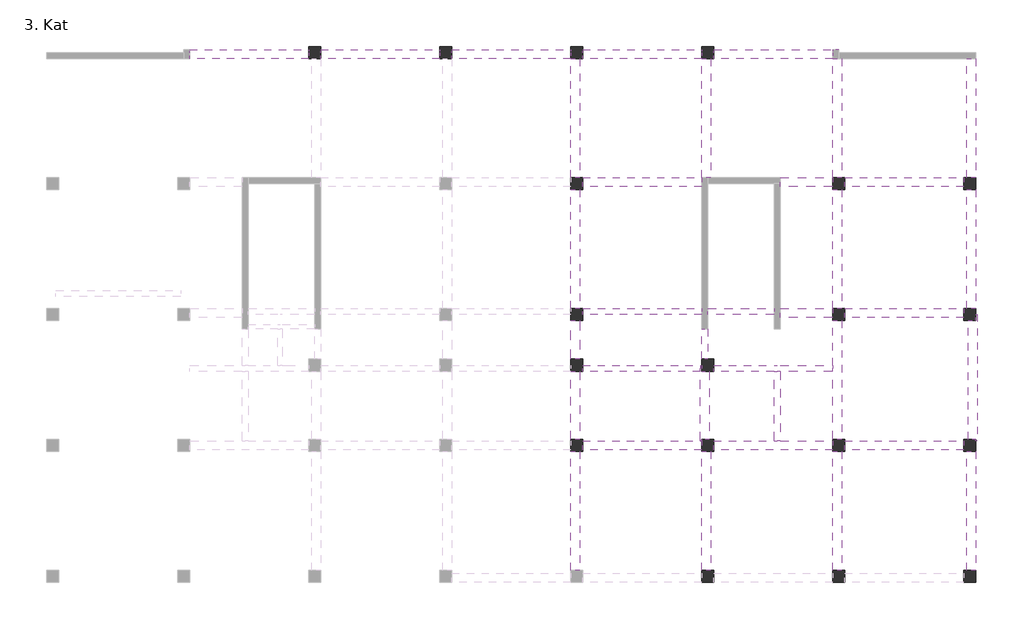
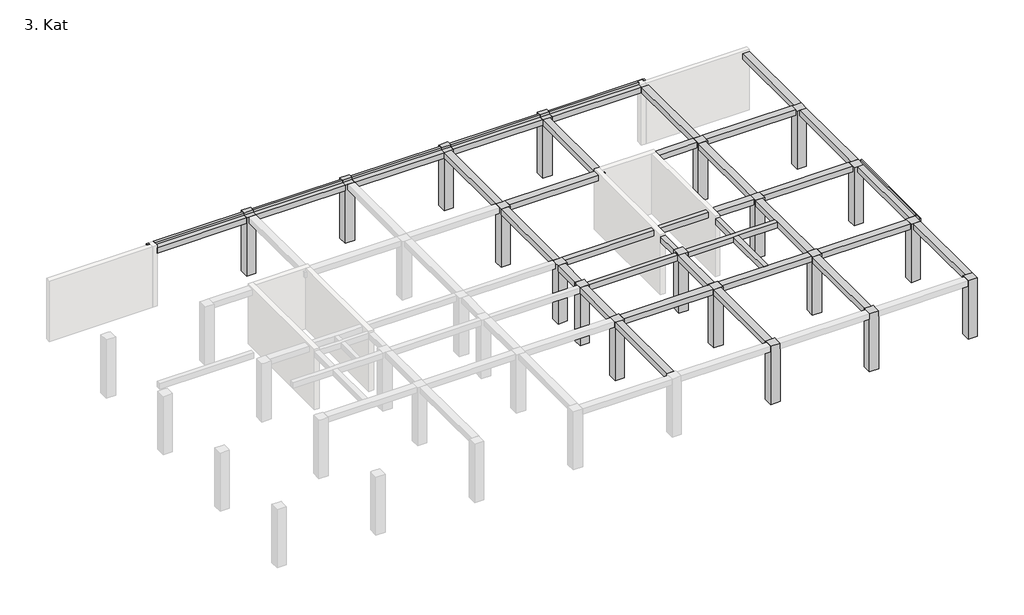
# One storey, part 2 of 2: 35 beams, 19 columns.
"""IFC4 building model written with IfcOpenShell, lengths in millimetres."""

from ifc_helpers import new_model, si_unit, frame, origin, place, context, project, spatial, polyline, outline, extrude, faceted_brep, element, save

model = new_model("IFC4")

# Units and contexts
model_context = context("Model", 3, world=origin())
ifc_project = project(units=[si_unit("LENGTHUNIT", "METRE", prefix="MILLI")], contexts=[model_context])

# Site, building, storey
site = spatial("IfcSite", under=ifc_project)
building = spatial("IfcBuilding", under=site)
storey = spatial("IfcBuildingStorey", under=building, Name="3. Kat", Elevation=15500.0)

# Beams
placement = place(None, origin())
element("IfcBeam", 1, ObjectType="M_Concrete-Rectangular Beam : 60x70cm kiriş", at=placement, inside=storey, context=model_context, shape_type="Brep", body=[
    faceted_brep([(16599.9993907, 34000.0004302, 21000.0), (16599.9993907, 34200.0000099, 21000.0), (8899.9995273, 34200.0000099, 21000.0), (8899.9995273, 34000.0004302, 21000.0), (8899.9993907, 33600.0000099, 20300.0), (16599.9993907, 33600.0000099, 20300.0), (16599.9993907, 33600.0000099, 20800.0), (8899.9993907, 33600.0000099, 20800.0), (8899.9995273, 34200.0000099, 20300.0), (16599.9993907, 34200.0000099, 20300.0), (8899.9993907, 34000.0004302, 20800.0), (16599.9993907, 34000.0004302, 20800.0)], [[[0, 1, 2, 3]], [[4, 5, 6, 7]], [[5, 4, 8, 9]], [[1, 9, 8, 2]], [[4, 7, 10, 3, 2, 8]], [[11, 10, 7, 6]], [[5, 9, 1, 0, 11, 6]], [[10, 11, 0, 3]]]),
    faceted_brep([(8299.9993907, 34200.0000099, 21000.0), (8299.9993907, 34200.0000099, 20300.0), (8299.9993907, 34000.0004302, 20300.0), (8299.9993907, 34000.0004302, 21000.0), (8499.9995273, 34000.0004302, 20300.0), (8499.9995273, 34000.0004302, 21000.0), (8499.9995273, 34200.0000099, 21000.0), (8499.9995273, 34200.0000099, 20300.0)], [[[0, 1, 2, 3]], [[3, 2, 4, 5]], [[6, 5, 4, 7]], [[0, 3, 5, 6]], [[2, 1, 7, 4]], [[1, 0, 6, 7]]]),
])
element("IfcBeam", 2, ObjectType="M_Concrete-Rectangular Beam : 60x70cm kiriş", at=placement, inside=storey, context=model_context, shape_type="SweptSolid", body=[
    extrude(outline(polyline([(34000.0004302, 21000.0), (34200.0000277, 21000.0), (34200.0000277, 20300.0), (33600.0000277, 20300.0), (33600.0000277, 20800.0), (34000.0004302, 20800.0), (34000.0004302, 21000.0)])), frame((17399.9993907, 0.0, 0.0), z_axis=(1.0, 0.0, 0.0), x_axis=(0.0, 1.0, 0.0)), (0.0, 0.0, 1.0), 7700.0),
])
element("IfcBeam", 3, ObjectType="M_Concrete-Rectangular Beam : 60x70cm kiriş", at=placement, inside=storey, context=model_context, shape_type="SweptSolid", body=[
    extrude(outline(polyline([(34000.0004302, 21000.0), (34200.000044, 21000.0), (34200.000044, 20300.0), (33600.000044, 20300.0), (33600.000044, 20800.0), (34000.0004302, 20800.0), (34000.0004302, 21000.0)])), frame((25899.9993907, 0.0, 0.0), z_axis=(1.0, 0.0, 0.0), x_axis=(0.0, 1.0, 0.0)), (0.0, 0.0, 1.0), 7700.0),
])
element("IfcBeam", 4, ObjectType="M_Concrete-Rectangular Beam : 60x70cm kiriş", at=placement, inside=storey, context=model_context, shape_type="SweptSolid", body=[
    extrude(outline(polyline([(34200.0000618, 21000.0), (34200.0000618, 20300.0), (33600.0000618, 20300.0), (33600.0000618, 20800.0), (34000.0004302, 20800.0), (34000.0004302, 21000.0), (34200.0000618, 21000.0)])), frame((34399.9993907, 0.0, 0.0), z_axis=(1.0, 0.0, 0.0), x_axis=(0.0, 1.0, 0.0)), (0.0, 0.0, 1.0), 7699.9999993),
])
element("IfcBeam", 5, ObjectType="M_Concrete-Rectangular Beam : 60x70cm kiriş", at=placement, inside=storey, context=model_context, shape_type="Brep", body=[
    faceted_brep([(50999.9994944, 34200.0000788, 21000.0), (42899.999681, 34200.0000788, 21000.0), (42899.999681, 34000.0004302, 21000.0), (50599.9994944, 34000.0004302, 21000.0), (50599.9994944, 34193.7257565, 21000.0), (50999.9994944, 34193.7257565, 21000.0), (50999.9994944, 34200.0000788, 20300.0), (42899.999681, 34200.0000788, 20300.0), (50999.9994944, 34193.7257565, 20300.0), (50599.9994944, 34193.7257565, 20300.0), (50599.9994944, 33600.0000788, 20300.0), (42899.999681, 33600.0000788, 20300.0), (42899.999681, 33600.0000788, 20800.0), (50599.9994944, 33600.0000788, 20800.0), (42899.999681, 34000.0004302, 20800.0), (50599.9994944, 34000.0004302, 20800.0)], [[[0, 1, 2, 3, 4, 5]], [[1, 0, 6, 7]], [[7, 6, 8, 9, 10, 11]], [[12, 11, 10, 13]], [[6, 0, 5, 8]], [[14, 12, 13, 15]], [[2, 14, 15, 3]], [[1, 7, 11, 12, 14, 2]], [[9, 4, 3, 15, 13, 10]], [[4, 9, 8, 5]]]),
])
element("IfcBeam", 6, ObjectType="M_Concrete-Rectangular Beam : 60x70cm kiriş", at=placement, inside=storey, context=model_context, shape_type="Brep", body=[
    faceted_brep([(33599.9994248, 33600.000044, 20800.0), (33599.9994248, 33600.000044, 20300.0), (33599.9994248, 25900.0003995, 20300.0), (33599.9994248, 25900.0003995, 20800.0), (34199.9994248, 33600.0009197, 20300.0), (34199.9994248, 25900.0004105, 20300.0), (34199.9994248, 25900.0004105, 20800.0), (34199.9994248, 33600.0009197, 20800.0)], [[[0, 1, 2, 3]], [[1, 4, 5, 2]], [[6, 5, 4, 7]], [[1, 0, 7, 4]], [[3, 2, 5, 6]], [[7, 0, 3, 6]]]),
])
element("IfcBeam", 7, ObjectType="M_Concrete-Rectangular Beam : 60x70cm kiriş", at=placement, inside=storey, context=model_context, shape_type="SweptSolid", body=[
    extrude(outline(polyline([(42699.9994393, 25300.0004179), (42499.9995162, 25300.0004179), (42499.9995162, 25500.0004459), (42699.9994393, 25500.0004459), (42699.9994393, 25300.0004179)])), frame((0.0, 0.0, 20300.0), z_axis=(0.0, 0.0, 1.0), x_axis=(1.0, 0.0, 0.0)), (0.0, 0.0, 1.0), 500.0),
    extrude(outline(polyline([(34399.9993907, 25300.0004179), (34399.9993907, 25900.0004179), (42099.9995162, 25900.0004179), (42099.9995162, 25300.0004179), (34399.9993907, 25300.0004179)])), frame((0.0, 0.0, 20300.0), z_axis=(0.0, 0.0, 1.0), x_axis=(1.0, 0.0, 0.0)), (0.0, 0.0, 1.0), 500.0),
])
element("IfcBeam", 8, ObjectType="M_Concrete-Rectangular Beam : 60x70cm kiriş", at=placement, inside=storey, context=model_context, shape_type="Brep", body=[
    faceted_brep([(42099.9994393, 25900.0004179, 20300.0), (42099.9994393, 25900.0004179, 20800.0), (42099.9994393, 33600.0000618, 20800.0), (42099.9994393, 33600.0000618, 20300.0), (42699.9994393, 25900.0004179, 20300.0), (42699.9994393, 33600.0009197, 20300.0), (42699.9994393, 25900.0004179, 20800.0), (42699.9994393, 33600.0009197, 20800.0)], [[[0, 1, 2, 3]], [[4, 0, 3, 5]], [[6, 4, 5, 7]], [[0, 4, 6, 1]], [[3, 2, 7, 5]], [[7, 2, 1, 6]]]),
])
element("IfcBeam", 9, ObjectType="M_Concrete-Rectangular Beam : 60x70cm kiriş", at=placement, inside=storey, context=model_context, shape_type="SweptSolid", body=[
    extrude(outline(polyline([(50599.9993899, 25900.0004722), (50599.9993899, 25300.0004722), (47199.999381, 25300.0004722), (47199.999381, 25900.0004722), (50599.9993899, 25900.0004722)])), frame((0.0, 0.0, 20300.0), z_axis=(0.0, 0.0, 1.0), x_axis=(1.0, 0.0, 0.0)), (0.0, 0.0, 1.0), 500.0),
])
element("IfcBeam", 10, ObjectType="M_Concrete-Rectangular Beam : 60x70cm kiriş", at=placement, inside=storey, context=model_context, shape_type="Brep", body=[
    faceted_brep([(50999.9994944, 34000.0004302, 21000.0), (51199.9994348, 34000.0004302, 21000.0), (51199.9994348, 34200.0000788, 21000.0), (50999.9994944, 34200.0000788, 21000.0), (50999.9994944, 34193.7257565, 21000.0), (51199.9994348, 34200.0000788, 20300.0), (51199.9994348, 34000.0004303, 20300.0), (50999.9994944, 34200.0000788, 20300.0), (50999.9994944, 34000.0004303, 20300.0), (50999.9994944, 34193.7257565, 20300.0)], [[[0, 1, 2, 3, 4]], [[5, 2, 1, 6]], [[7, 5, 6, 8, 9]], [[2, 5, 7, 3]], [[8, 0, 4, 3, 7, 9]], [[1, 0, 8, 6]]]),
    faceted_brep([(50599.9994348, 33600.0000788, 20800.0), (50599.9994348, 33600.0000788, 20300.0), (50599.9994348, 25900.0004722, 20300.0), (50599.9994348, 25900.0004722, 20800.0), (51199.9994348, 33600.0000788, 20800.0), (51199.9994348, 33600.0000788, 20300.0), (51199.9994348, 25900.0004722, 20300.0), (51199.9994348, 25900.0004722, 20800.0)], [[[0, 1, 2, 3]], [[1, 0, 4, 5]], [[3, 2, 6, 7]], [[4, 0, 3, 7]], [[7, 6, 5, 4]], [[1, 5, 6, 2]]]),
])
element("IfcBeam", 11, ObjectType="M_Concrete-Rectangular Beam : 60x70cm kiriş", at=placement, inside=storey, context=model_context, shape_type="SweptSolid", body=[
    extrude(outline(polyline([(59100.0000836, 25300.0000972), (51399.9996879, 25300.0000972), (51399.9996879, 25900.0000972), (59100.0000836, 25900.0000972), (59100.0000836, 25300.0000972)])), frame((0.0, 0.0, 20300.0), z_axis=(0.0, 0.0, 1.0), x_axis=(1.0, 0.0, 0.0)), (0.0, 0.0, 1.0), 500.0),
])
element("IfcBeam", 12, ObjectType="M_Concrete-Rectangular Beam : 60x70cm kiriş", at=placement, inside=storey, context=model_context, shape_type="SweptSolid", body=[
    extrude(outline(polyline([(59899.9996867, 25900.0004522), (59299.9996867, 25900.0004522), (59299.9996867, 33600.0004303), (59899.9996867, 33600.0004303), (59899.9996867, 25900.0004522)])), frame((0.0, 0.0, 20300.0), z_axis=(0.0, 0.0, 1.0), x_axis=(1.0, 0.0, 0.0)), (0.0, 0.0, 1.0), 500.0),
])
element("IfcBeam", 13, ObjectType="M_Concrete-Rectangular Beam : 60x70cm kiriş", at=placement, inside=storey, context=model_context, shape_type="SweptSolid", body=[
    extrude(outline(polyline([(33599.9994953, 25100.0004105), (34199.9994953, 25100.0004105), (34199.9994953, 17400.0009197), (33599.9994953, 17400.0009197), (33599.9994953, 25100.0004105)])), frame((0.0, 0.0, 20300.0), z_axis=(0.0, 0.0, 1.0), x_axis=(1.0, 0.0, 0.0)), (0.0, 0.0, 1.0), 500.0),
])
element("IfcBeam", 14, ObjectType="M_Concrete-Rectangular Beam : 40x70cm kiriş 2", at=placement, inside=storey, context=model_context, shape_type="SweptSolid", body=[
    extrude(outline(polyline([(42099.9995162, 16050.0004138), (42499.9995162, 16050.0004138), (42499.9995162, 14100.0003816), (42099.9995162, 14100.0003816), (42099.9995162, 16050.0004138)])), frame((0.0, 0.0, 20300.0), z_axis=(0.0, 0.0, 1.0), x_axis=(1.0, 0.0, 0.0)), (0.0, 0.0, 1.0), 500.0),
])
element("IfcBeam", 15, ObjectType="M_Concrete-Rectangular Beam : 40x70cm kiriş 2", at=placement, inside=storey, context=model_context, shape_type="SweptSolid", body=[
    extrude(outline(polyline([(41999.9997966, 13700.0003995), (41999.9997966, 13300.0003995), (34399.9997415, 13300.0003995), (34399.9997415, 13700.0003995), (41999.9997966, 13700.0003995)])), frame((0.0, 0.0, 20300.0), z_axis=(0.0, 0.0, 1.0), x_axis=(1.0, 0.0, 0.0)), (0.0, 0.0, 1.0), 500.0),
])
element("IfcBeam", 16, ObjectType="M_Concrete-Rectangular Beam : 40x70cm kiriş 2", at=placement, inside=storey, context=model_context, shape_type="SweptSolid", body=[
    extrude(outline(polyline([(34399.9993907, 17000.0007895), (34399.9993907, 17400.0007895), (42099.9995162, 17400.0007895), (42099.9995162, 17000.0007895), (34399.9993907, 17000.0007895)])), frame((0.0, 0.0, 20300.0), z_axis=(0.0, 0.0, 1.0), x_axis=(1.0, 0.0, 0.0)), (0.0, 0.0, 1.0), 500.0),
])
element("IfcBeam", 17, ObjectType="M_Concrete-Rectangular Beam : 40x70cm kiriş 2", at=placement, inside=storey, context=model_context, shape_type="SweptSolid", body=[
    extrude(outline(polyline([(42499.9995162, 17000.0003766), (42499.9995162, 17400.0003766), (46799.999381, 17400.0003766), (46799.999381, 17000.0003766), (42499.9995162, 17000.0003766)])), frame((0.0, 0.0, 20300.0), z_axis=(0.0, 0.0, 1.0), x_axis=(1.0, 0.0, 0.0)), (0.0, 0.0, 1.0), 500.0),
])
element("IfcBeam", 18, ObjectType="M_Concrete-Rectangular Beam : 60x70cm kiriş", at=placement, inside=storey, context=model_context, shape_type="SweptSolid", body=[
    extrude(outline(polyline([(33599.9997451, 14100.0003995), (33599.9997451, 16599.9999518), (34199.9997451, 16599.9999518), (34199.9997451, 14100.0003995), (33599.9997451, 14100.0003995)])), frame((0.0, 0.0, 20300.0), z_axis=(0.0, 0.0, 1.0), x_axis=(1.0, 0.0, 0.0)), (0.0, 0.0, 1.0), 500.0),
])
element("IfcBeam", 19, ObjectType="M_Concrete-Rectangular Beam : 40x70cm kiriş 2", at=placement, inside=storey, context=model_context, shape_type="Brep", body=[
    faceted_brep([(42899.9990901, 13300.0003995, 20300.0), (46799.999381, 13300.0003995, 20300.0), (47199.999381, 13300.0003995, 20300.0), (50599.9996909, 13300.0003995, 20300.0), (50599.9996909, 13300.0003995, 20800.0), (47199.999381, 13300.0003995, 20800.0), (46799.999381, 13300.0003995, 20800.0), (42899.9990901, 13300.0003995, 20800.0), (42899.9990901, 13700.0003995, 20300.0), (46799.999381, 13700.0003995, 20300.0), (47199.999381, 13700.0003995, 20300.0), (50599.9996909, 13700.0003995, 20300.0), (42899.9990901, 13700.0003995, 20800.0), (46799.999381, 13700.0003995, 20800.0), (47199.999381, 13700.0003995, 20800.0), (50599.9996909, 13700.0003995, 20800.0)], [[[0, 1, 2, 3, 4, 5, 6, 7]], [[3, 2, 1, 0, 8, 9, 10, 11]], [[11, 10, 9, 8, 12, 13, 14, 15]], [[3, 11, 15, 4]], [[7, 6, 5, 4, 15, 14, 13, 12]], [[8, 0, 7, 12]]]),
])
element("IfcBeam", 20, ObjectType="M_Concrete-Rectangular Beam : 40x70cm kiriş 2", at=placement, inside=storey, context=model_context, shape_type="SweptSolid", body=[
    extrude(outline(polyline([(46799.999381, 16050.0004138), (47199.999381, 16050.0004138), (47199.999381, 13700.0003995), (46799.999381, 13700.0003995), (46799.999381, 16050.0004138)])), frame((0.0, 0.0, 20300.0), z_axis=(0.0, 0.0, 1.0), x_axis=(1.0, 0.0, 0.0)), (0.0, 0.0, 1.0), 500.0),
    extrude(outline(polyline([(46799.999381, 13300.0003995), (47199.999381, 13300.0003995), (47199.999381, 8800.0009197), (46799.999381, 8800.0009197), (46799.999381, 13300.0003995)])), frame((0.0, 0.0, 20300.0), z_axis=(0.0, 0.0, 1.0), x_axis=(1.0, 0.0, 0.0)), (0.0, 0.0, 1.0), 500.0),
])
element("IfcBeam", 21, ObjectType="M_Concrete-Rectangular Beam : 60x70cm kiriş", at=placement, inside=storey, context=model_context, shape_type="Brep", body=[
    faceted_brep([(34399.9993907, 8200.0009197, 20800.0), (34399.9993907, 8200.0009197, 20300.0), (42099.9993899, 8200.0009197, 20300.0), (42099.9993899, 8200.0009197, 20800.0), (34399.9993907, 8800.0009197, 20300.0), (41999.9997966, 8800.0009197, 20300.0), (42099.9993899, 8800.0009197, 20300.0), (34399.9993907, 8800.0009197, 20800.0), (41999.9997966, 8800.0009197, 20800.0), (42099.9993899, 8800.0009197, 20800.0)], [[[0, 1, 2, 3]], [[1, 4, 5, 6, 2]], [[4, 7, 8, 9, 6, 5]], [[7, 0, 3, 9, 8]], [[1, 0, 7, 4]], [[3, 2, 6, 9]]]),
])
element("IfcBeam", 22, ObjectType="M_Concrete-Rectangular Beam : 60x70cm kiriş", at=placement, inside=storey, context=model_context, shape_type="Brep", body=[
    faceted_brep([(50599.9993899, 8200.0009197, 20300.0), (50599.9993899, 8200.0009197, 20800.0), (42899.9993899, 8200.0009197, 20800.0), (42899.9993899, 8200.0009197, 20300.0), (50599.9993899, 8800.0009197, 20300.0), (42899.9993899, 8800.0009197, 20300.0), (46799.999381, 8800.0009197, 20300.0), (47199.999381, 8800.0009197, 20300.0), (50599.9993899, 8800.0009197, 20800.0), (42899.9993899, 8800.0009197, 20800.0), (46799.999381, 8800.0009197, 20800.0), (47199.999381, 8800.0009197, 20800.0)], [[[0, 1, 2, 3]], [[4, 0, 3, 5, 6, 7]], [[8, 4, 7, 6, 5, 9, 10, 11]], [[1, 8, 11, 10, 9, 2]], [[1, 0, 4, 8]], [[3, 2, 9, 5]]]),
])
element("IfcBeam", 23, ObjectType="M_Concrete-Rectangular Beam : 60x70cm kiriş", at=placement, inside=storey, context=model_context, shape_type="Brep", body=[
    faceted_brep([(42599.9997966, 8900.0009197, 20800.0), (42599.9997966, 8900.0009197, 20300.0), (42599.9997966, 13300.0003816, 20300.0), (42599.9997966, 13300.0003816, 20800.0), (41999.9997966, 8800.0009197, 20300.0), (41999.9997966, 13300.0003995, 20300.0), (41999.9997966, 13700.0003995, 20300.0), (42099.9993899, 13700.0003995, 20300.0), (42099.9993899, 13300.0003816, 20300.0), (42099.9993899, 8900.0009197, 20300.0), (42099.9993899, 8800.0009197, 20300.0), (41999.9997966, 8800.0009197, 20800.0), (41999.9997966, 13300.0003995, 20800.0), (41999.9997966, 13700.0003995, 20800.0), (42099.9993899, 8800.0009197, 20800.0), (42099.9993899, 8900.0009197, 20800.0), (42099.9993899, 13300.0003816, 20800.0), (42099.9993899, 13700.0003995, 20800.0)], [[[0, 1, 2, 3]], [[4, 5, 6, 7, 8, 2, 1, 9, 10]], [[4, 11, 12, 13, 6, 5]], [[11, 4, 10, 14]], [[13, 12, 11, 14, 15, 0, 3, 16, 17]], [[6, 13, 17, 7]], [[9, 15, 14, 10]], [[15, 9, 1, 0]], [[8, 16, 3, 2]], [[16, 8, 7, 17]]]),
])
element("IfcBeam", 24, ObjectType="M_Concrete-Rectangular Beam : 60x70cm kiriş", at=placement, inside=storey, context=model_context, shape_type="SweptSolid", body=[
    extrude(outline(polyline([(34199.9994953, 8900.0009197), (33599.9994953, 8900.0009197), (33599.9994953, 13300.0003995), (34199.9994953, 13300.0003995), (34199.9994953, 8900.0009197)])), frame((0.0, 0.0, 20300.0), z_axis=(0.0, 0.0, 1.0), x_axis=(1.0, 0.0, 0.0)), (0.0, 0.0, 1.0), 500.0),
])
element("IfcBeam", 25, ObjectType="M_Concrete-Rectangular Beam : 60x70cm kiriş", at=placement, inside=storey, context=model_context, shape_type="SweptSolid", body=[
    extrude(outline(polyline([(47199.999381, 16800.0008288), (47199.999381, 17400.0008288), (50599.9993899, 17400.0008288), (50599.9993899, 16800.0008288), (47199.999381, 16800.0008288)])), frame((0.0, 0.0, 20300.0), z_axis=(0.0, 0.0, 1.0), x_axis=(1.0, 0.0, 0.0)), (0.0, 0.0, 1.0), 500.0),
])
element("IfcBeam", 26, ObjectType="M_Concrete-Rectangular Beam : 60x70cm kiriş", at=placement, inside=storey, context=model_context, shape_type="Brep", body=[
    faceted_brep([(50599.999688, 17400.0008288, 20300.0), (50599.999688, 17400.0008288, 20800.0), (50599.999688, 25099.9999414, 20800.0), (50599.999688, 25099.9999414, 20300.0), (51199.999688, 17400.0009197, 20300.0), (51199.999688, 25099.9999414, 20300.0), (51199.999688, 25099.9999414, 20800.0), (51199.999688, 17400.0009197, 20800.0)], [[[0, 1, 2, 3]], [[4, 0, 3, 5]], [[5, 6, 7, 4]], [[4, 7, 1, 0]], [[2, 1, 7, 6]], [[5, 3, 2, 6]]]),
])
element("IfcBeam", 27, ObjectType="M_Concrete-Rectangular Beam : 60x70cm kiriş", at=placement, inside=storey, context=model_context, shape_type="SweptSolid", body=[
    extrude(outline(polyline([(59299.9997153, 17400.0009197), (59299.9997153, 25099.9999188), (59899.9997153, 25099.9999188), (59899.9997153, 17400.0009197), (59299.9997153, 17400.0009197)])), frame((0.0, 0.0, 20300.0), z_axis=(0.0, 0.0, 1.0), x_axis=(1.0, 0.0, 0.0)), (0.0, 0.0, 1.0), 500.0),
])
element("IfcBeam", 28, ObjectType="M_Concrete-Rectangular Beam : 60x70cm kiriş", at=placement, inside=storey, context=model_context, shape_type="SweptSolid", body=[
    extrude(outline(polyline([(51399.9993899, 17399.9995872), (59100.0000836, 17399.9995872), (59100.0000836, 16799.9995872), (51399.9993899, 16799.9995872), (51399.9993899, 17399.9995872)])), frame((0.0, 0.0, 20300.0), z_axis=(0.0, 0.0, 1.0), x_axis=(1.0, 0.0, 0.0)), (0.0, 0.0, 1.0), 500.0),
])
element("IfcBeam", 29, ObjectType="M_Concrete-Rectangular Beam : 60x70cm kiriş", at=placement, inside=storey, context=model_context, shape_type="Brep", body=[
    faceted_brep([(50599.9996909, 16600.0009197, 20300.0), (50599.9996909, 13700.0003995, 20300.0), (50599.9996909, 13300.0003995, 20300.0), (50599.9996909, 8900.000455, 20300.0), (50599.9996909, 8900.000455, 20800.0), (50599.9996909, 13300.0003995, 20800.0), (50599.9996909, 13700.0003995, 20800.0), (50599.9996909, 16600.0009197, 20800.0), (51199.9996909, 16600.0009197, 20300.0), (51199.9996909, 8900.000455, 20300.0), (51199.9996909, 16600.0009197, 20800.0), (51199.9996909, 8900.000455, 20800.0)], [[[0, 1, 2, 3, 4, 5, 6, 7]], [[3, 2, 1, 0, 8, 9]], [[9, 8, 10, 11]], [[7, 6, 5, 4, 11, 10]], [[3, 9, 11, 4]], [[8, 0, 7, 10]]]),
])
element("IfcBeam", 30, ObjectType="M_Concrete-Rectangular Beam : 60x70cm kiriş", at=placement, inside=storey, context=model_context, shape_type="Brep", body=[
    faceted_brep([(59899.9997758, 8800.0009197, 21000.0), (59899.9997758, 8200.0009197, 21000.0), (59999.9993848, 8200.0009197, 21000.0), (59999.9993848, 8800.0009197, 21000.0), (59900.0000836, 8200.0009197, 20300.0), (59999.9993848, 8200.0009197, 20300.0), (59999.9993848, 8800.0009197, 20300.0), (59900.0000836, 8800.0009197, 20300.0)], [[[0, 1, 2, 3]], [[1, 4, 5, 2]], [[6, 5, 4, 7]], [[7, 0, 3, 6]], [[1, 0, 7, 4]], [[3, 2, 5, 6]]]),
    faceted_brep([(51399.9993899, 8800.0009197, 20800.0), (51399.9993899, 8200.0009197, 20800.0), (59100.0000836, 8200.0009197, 20800.0), (59100.0000836, 8800.0009197, 20800.0), (51399.9993899, 8800.0009197, 20300.0), (51399.9993899, 8200.0009197, 20300.0), (59100.0000836, 8200.0009197, 20300.0), (59100.0000836, 8800.0009197, 20300.0)], [[[0, 1, 2, 3]], [[4, 5, 1, 0]], [[2, 6, 7, 3]], [[1, 5, 6, 2]], [[5, 4, 7, 6]], [[4, 0, 3, 7]]]),
])
element("IfcBeam", 31, ObjectType="M_Concrete-Rectangular Beam : 60x70cm kiriş", at=placement, inside=storey, context=model_context, shape_type="Brep", body=[
    faceted_brep([(59899.9997758, 17000.0009197, 21000.0), (59899.9997758, 8800.0009197, 21000.0), (59999.9993848, 8800.0009197, 21000.0), (59999.9993848, 17000.0009197, 21000.0), (59999.9993848, 8800.0009197, 20300.0), (59999.9993848, 17000.0009197, 20300.0), (59900.0000836, 8800.0009197, 20300.0), (59900.0000836, 8900.0009197, 20300.0), (59399.9993848, 8900.0009197, 20300.0), (59399.9993848, 16600.0009197, 20300.0), (59900.0000836, 16600.0009197, 20300.0), (59900.0000836, 17000.0009197, 20300.0), (59399.9993848, 8900.0009197, 20800.0), (59399.9993848, 16600.0009197, 20800.0), (59899.9997758, 8900.0009197, 20800.0), (59899.9997758, 16600.0009197, 20800.0)], [[[0, 1, 2, 3]], [[2, 4, 5, 3]], [[5, 4, 6, 7, 8, 9, 10, 11]], [[8, 12, 13, 9]], [[4, 2, 1, 6]], [[12, 14, 15, 13]], [[11, 10, 15, 14, 7, 6, 1, 0]], [[3, 5, 11, 0]], [[7, 14, 12, 8]], [[15, 10, 9, 13]]]),
])
element("IfcBeam", 32, ObjectType="M_Concrete-Rectangular Beam : 60x70cm kiriş", at=placement, inside=storey, context=model_context, shape_type="SweptSolid", body=[
    extrude(outline(polyline([(59899.9997503, 400.0009197), (59299.9997503, 400.0009197), (59299.9997503, 8100.0009197), (59899.9997503, 8100.0009197), (59899.9997503, 400.0009197)])), frame((0.0, 0.0, 20300.0), z_axis=(0.0, 0.0, 1.0), x_axis=(1.0, 0.0, 0.0)), (0.0, 0.0, 1.0), 500.0),
])
element("IfcBeam", 33, ObjectType="M_Concrete-Rectangular Beam : 60x70cm kiriş", at=placement, inside=storey, context=model_context, shape_type="SweptSolid", body=[
    extrude(outline(polyline([(51199.999723, 400.0009197), (50599.999723, 400.0009197), (50599.999723, 8100.0009197), (51199.999723, 8100.0009197), (51199.999723, 400.0009197)])), frame((0.0, 0.0, 20300.0), z_axis=(0.0, 0.0, 1.0), x_axis=(1.0, 0.0, 0.0)), (0.0, 0.0, 1.0), 500.0),
])
element("IfcBeam", 34, ObjectType="M_Concrete-Rectangular Beam : 60x70cm kiriş", at=placement, inside=storey, context=model_context, shape_type="SweptSolid", body=[
    extrude(outline(polyline([(42699.999723, 400.0009197), (42099.999723, 400.0009197), (42099.999723, 8100.0009197), (42699.999723, 8100.0009197), (42699.999723, 400.0009197)])), frame((0.0, 0.0, 20300.0), z_axis=(0.0, 0.0, 1.0), x_axis=(1.0, 0.0, 0.0)), (0.0, 0.0, 1.0), 500.0),
])
element("IfcBeam", 35, ObjectType="M_Concrete-Rectangular Beam : 60x70cm kiriş", at=placement, inside=storey, context=model_context, shape_type="SweptSolid", body=[
    extrude(outline(polyline([(33599.9997451, 400.0004179), (33599.9997451, 8100.0004174), (34199.9997451, 8100.0004174), (34199.9997451, 400.0004179), (33599.9997451, 400.0004179)])), frame((0.0, 0.0, 20300.0), z_axis=(0.0, 0.0, 1.0), x_axis=(1.0, 0.0, 0.0)), (0.0, 0.0, 1.0), 500.0),
])

# Columns
element("IfcColumn", 36, ObjectType="M_Concrete-Rectangular-Column : 80x80cm kolon", at=placement, inside=storey, context=model_context, shape_type="Brep", body=[
    faceted_brep([(34399.9993907, 8900.0009197, 15500.0), (34399.9993907, 8100.0009197, 15500.0), (33599.9993907, 8100.0009197, 15500.0), (33599.9993907, 8900.0009197, 15500.0), (34399.9993907, 8900.0009197, 20800.0), (34399.9993907, 8800.0009197, 20800.0), (34399.9993907, 8200.0009197, 20800.0), (34399.9993907, 8100.0009197, 20800.0), (34199.9997451, 8100.0009197, 20800.0), (33599.9993907, 8100.0009197, 20800.0), (33599.9993907, 8200.0009197, 20800.0), (33599.9993907, 8800.0009197, 20800.0), (33599.9993907, 8900.0009197, 20800.0), (34199.9994953, 8900.0009197, 20800.0)], [[[0, 1, 2, 3]], [[1, 0, 4, 5, 6, 7]], [[2, 1, 7, 8, 9]], [[3, 2, 9, 10, 11, 12]], [[0, 3, 12, 13, 4]], [[7, 6, 5, 4, 13, 12, 11, 10, 9, 8]]]),
])
element("IfcColumn", 37, ObjectType="M_Concrete-Rectangular-Column : 80x80cm kolon", at=placement, inside=storey, context=model_context, shape_type="Brep", body=[
    faceted_brep([(34399.9993907, 14100.0003995, 15500.0), (34399.9993907, 13300.0003995, 15500.0), (33599.9993907, 13300.0003995, 15500.0), (33599.9993907, 14100.0003995, 15500.0), (34399.9993907, 14100.0003995, 20800.0), (34399.9993907, 13700.0003995, 20800.0), (34399.9993907, 13300.0003995, 20800.0), (34399.9993907, 13300.0003995, 20300.0), (34199.9994953, 13300.0003995, 20800.0), (33599.9993907, 13300.0003995, 20800.0), (33599.9993907, 13300.0003995, 20300.0), (33599.9993907, 13700.0003995, 20800.0), (33599.9993907, 14100.0003995, 20800.0), (34199.9997451, 14100.0003995, 20800.0)], [[[0, 1, 2, 3]], [[1, 0, 4, 5, 6, 7]], [[2, 1, 7, 6, 8, 9, 10]], [[3, 2, 10, 9, 11, 12]], [[0, 3, 12, 13, 4]], [[6, 5, 4, 13, 12, 11, 9, 8]]]),
])
element("IfcColumn", 38, ObjectType="M_Concrete-Rectangular-Column : 80x80cm kolon", at=placement, inside=storey, context=model_context, shape_type="Brep", body=[
    faceted_brep([(34399.9993907, 17400.0009197, 15500.0), (34399.9993907, 16600.0009197, 15500.0), (33599.9993907, 16600.0009197, 15500.0), (33599.9993907, 17400.0009197, 15500.0), (34399.9993907, 17400.0009197, 20800.0), (34399.9993907, 17000.0007895, 20800.0), (34399.9993907, 16600.0009197, 20800.0), (34199.9997451, 16600.0009197, 20800.0), (33599.9993907, 16600.0009197, 20800.0), (33599.9993907, 17000.0007711, 20800.0), (33599.9993907, 17400.0009197, 20800.0), (34199.9994953, 17400.0009197, 20800.0)], [[[0, 1, 2, 3]], [[1, 0, 4, 5, 6]], [[2, 1, 6, 7, 8]], [[3, 2, 8, 9, 10]], [[0, 3, 10, 11, 4]], [[6, 5, 4, 11, 10, 9, 8, 7]]]),
])
element("IfcColumn", 39, ObjectType="M_Concrete-Rectangular-Column : 80x80cm kolon", at=placement, inside=storey, context=model_context, shape_type="Brep", body=[
    faceted_brep([(34399.9993907, 25900.0004105, 15500.0), (34399.9993907, 25100.0004105, 15500.0), (33599.9993907, 25100.0004105, 15500.0), (33599.9993907, 25900.0004105, 15500.0), (34399.9993907, 25900.0004105, 20800.0), (34399.9993907, 25300.0004179, 20800.0), (34399.9993907, 25100.0004105, 20800.0), (34199.9994953, 25100.0004105, 20800.0), (33599.9993907, 25100.0004105, 20800.0), (33599.9993907, 25300.0003995, 20800.0), (33599.9993907, 25900.0004105, 20800.0), (34199.9994248, 25900.0004105, 20800.0)], [[[0, 1, 2, 3]], [[1, 0, 4, 5, 6]], [[2, 1, 6, 7, 8]], [[3, 2, 8, 9, 10]], [[0, 3, 10, 11, 4]], [[6, 5, 4, 11, 10, 9, 8, 7]]]),
])
element("IfcColumn", 40, ObjectType="M_Concrete-Rectangular-Column : 80x80cm kolon", at=placement, inside=storey, context=model_context, shape_type="Brep", body=[
    faceted_brep([(34399.9993907, 34400.0009197, 15500.0), (34399.9993907, 33600.0009197, 15500.0), (33599.9993907, 33600.0009197, 15500.0), (33599.9993907, 34400.0009197, 15500.0), (34399.9993907, 34400.0009197, 21000.0), (34399.9993907, 34200.0000618, 21000.0), (34399.9993907, 34000.0004302, 21000.0), (34399.9993907, 34000.0004302, 20800.0), (34399.9993907, 33600.0009197, 20800.0), (34199.9994248, 33600.0009197, 20800.0), (33599.9993907, 33600.0009197, 20800.0), (33599.9993907, 34000.0004302, 20800.0), (33599.9993907, 34000.0004302, 21000.0), (33599.9993907, 34200.000044, 21000.0), (33599.9993907, 34400.0009197, 21000.0)], [[[0, 1, 2, 3]], [[1, 0, 4, 5, 6, 7, 8]], [[2, 1, 8, 9, 10]], [[3, 2, 10, 11, 12, 13, 14]], [[0, 3, 14, 4]], [[4, 14, 13, 12, 6, 5]], [[7, 11, 10, 9, 8]], [[11, 7, 6, 12]]]),
])
element("IfcColumn", 41, ObjectType="M_Concrete-Rectangular-Column : 80x80cm kolon", at=placement, inside=storey, context=model_context, shape_type="Brep", body=[
    faceted_brep([(25899.9993907, 34400.0009197, 15500.0), (25899.9993907, 33600.0009197, 15500.0), (25099.9993907, 33600.0009197, 15500.0), (25099.9993907, 34400.0009197, 15500.0), (25899.9993907, 34400.0009197, 21000.0), (25899.9993907, 34200.000044, 21000.0), (25899.9993907, 34000.0004302, 21000.0), (25899.9993907, 34000.0004302, 20800.0), (25899.9993907, 33600.0009197, 20800.0), (25299.9996503, 33600.0009197, 20800.0), (25099.9993907, 33600.0009197, 20800.0), (25099.9993907, 34000.0004302, 20800.0), (25099.9993907, 34000.0004302, 21000.0), (25099.9993907, 34200.0000277, 21000.0), (25099.9993907, 34400.0009197, 21000.0)], [[[0, 1, 2, 3]], [[1, 0, 4, 5, 6, 7, 8]], [[2, 1, 8, 9, 10]], [[3, 2, 10, 11, 12, 13, 14]], [[0, 3, 14, 4]], [[4, 14, 13, 12, 6, 5]], [[7, 11, 10, 9, 8]], [[11, 7, 6, 12]]]),
])
element("IfcColumn", 42, ObjectType="M_Concrete-Rectangular-Column : 80x80cm kolon", at=placement, inside=storey, context=model_context, shape_type="Brep", body=[
    faceted_brep([(17399.9993907, 34400.0009197, 15500.0), (17399.9993907, 33600.0009197, 15500.0), (16599.9993907, 33600.0009197, 15500.0), (16599.9993907, 34400.0009197, 15500.0), (17399.9993907, 34400.0009197, 21000.0), (17399.9993907, 34200.0000277, 21000.0), (17399.9993907, 34000.0004302, 21000.0), (17399.9993907, 34000.0004302, 20800.0), (17399.9993907, 33600.0009197, 20800.0), (16799.9996817, 33600.0009197, 20800.0), (16599.9993907, 33600.0009197, 20800.0), (16599.9993907, 34000.0004302, 20800.0), (16599.9993907, 34000.0004302, 21000.0), (16599.9993907, 34200.0000099, 21000.0), (16599.9993907, 34400.0009197, 21000.0)], [[[0, 1, 2, 3]], [[1, 0, 4, 5, 6, 7, 8]], [[2, 1, 8, 9, 10]], [[3, 2, 10, 11, 12, 13, 14]], [[0, 3, 14, 4]], [[4, 14, 13, 12, 6, 5]], [[7, 11, 10, 9, 8]], [[11, 7, 6, 12]]]),
])
element("IfcColumn", 43, ObjectType="M_Concrete-Rectangular-Column : 80x80cm kolon", at=placement, inside=storey, context=model_context, shape_type="Brep", body=[
    faceted_brep([(42899.9993899, 400.0009197, 15500.0), (42899.9993899, -399.9990803, 15500.0), (42099.9993899, -399.9990803, 15500.0), (42099.9993899, 400.0009197, 15500.0), (42899.9993899, 400.0009197, 20800.0), (42899.9993899, 200.0003118, 20800.0), (42899.9993899, -399.9990803, 20800.0), (42099.9993899, -399.9990803, 20800.0), (42099.9993899, 200.0003118, 20800.0), (42099.9993899, 400.0009197, 20800.0), (42699.999723, 400.0009197, 20800.0)], [[[0, 1, 2, 3]], [[1, 0, 4, 5, 6]], [[2, 1, 6, 7]], [[3, 2, 7, 8, 9]], [[0, 3, 9, 10, 4]], [[6, 5, 4, 10, 9, 8, 7]]]),
])
element("IfcColumn", 44, ObjectType="M_Concrete-Rectangular-Column : 80x80cm kolon", at=placement, inside=storey, context=model_context, shape_type="Brep", body=[
    faceted_brep([(51399.9993899, 400.0009197, 15500.0), (51399.9993899, -399.9990803, 15500.0), (50599.9993899, -399.9990803, 15500.0), (50599.9993899, 400.0009197, 15500.0), (51399.9993899, 400.0009197, 20800.0), (51399.9993899, 200.0003118, 20800.0), (51399.9993899, -399.9990803, 20800.0), (50599.9993899, -399.9990803, 20800.0), (50599.9993899, 200.0003118, 20800.0), (50599.9993899, 400.0009197, 20800.0), (51199.999723, 400.0009197, 20800.0)], [[[0, 1, 2, 3]], [[1, 0, 4, 5, 6]], [[2, 1, 6, 7]], [[3, 2, 7, 8, 9]], [[0, 3, 9, 10, 4]], [[6, 5, 4, 10, 9, 8, 7]]]),
])
element("IfcColumn", 45, ObjectType="M_Concrete-Rectangular-Column : 80x80cm kolon", at=placement, inside=storey, context=model_context, shape_type="Brep", body=[
    faceted_brep([(59900.0000836, 400.0009197, 15500.0), (59900.0000836, -399.9990803, 15500.0), (59100.0000836, -399.9990803, 15500.0), (59100.0000836, 400.0009197, 15500.0), (59900.0000836, 400.0009197, 20800.0), (59900.0000836, -399.9990803, 20800.0), (59100.0000836, -399.9990803, 20800.0), (59100.0000836, 200.0003118, 20800.0), (59100.0000836, 400.0009197, 20800.0), (59299.9997503, 400.0009197, 20800.0)], [[[0, 1, 2, 3]], [[1, 0, 4, 5]], [[2, 1, 5, 6]], [[3, 2, 6, 7, 8]], [[0, 3, 8, 9, 4]], [[5, 4, 9, 8, 7, 6]]]),
])
element("IfcColumn", 46, ObjectType="M_Concrete-Rectangular-Column : 80x80cm kolon", at=placement, inside=storey, context=model_context, shape_type="Brep", body=[
    faceted_brep([(59900.0000836, 8900.0009197, 15500.0), (59900.0000836, 8100.0009197, 15500.0), (59100.0000836, 8100.0009197, 15500.0), (59100.0000836, 8900.0009197, 15500.0), (59900.0000836, 8900.0009197, 20300.0), (59900.0000836, 8900.0009197, 20800.0), (59900.0000836, 8100.0009197, 20800.0), (59299.9997503, 8100.0009197, 20800.0), (59100.0000836, 8100.0009197, 20800.0), (59100.0000836, 8200.0009197, 20800.0), (59100.0000836, 8800.0009197, 20800.0), (59100.0000836, 8900.0009197, 20800.0), (59399.9993848, 8900.0009197, 20800.0)], [[[0, 1, 2, 3]], [[1, 0, 4, 5, 6]], [[2, 1, 6, 7, 8]], [[3, 2, 8, 9, 10, 11]], [[0, 3, 11, 12, 5, 4]], [[6, 5, 12, 11, 10, 9, 8, 7]]]),
])
element("IfcColumn", 47, ObjectType="M_Concrete-Rectangular-Column : 80x80cm kolon", at=placement, inside=storey, context=model_context, shape_type="Brep", body=[
    faceted_brep([(51399.9993899, 8900.0009197, 15500.0), (51399.9993899, 8100.0009197, 15500.0), (50599.9993899, 8100.0009197, 15500.0), (50599.9993899, 8900.0009197, 15500.0), (51399.9993899, 8900.0009197, 20800.0), (51399.9993899, 8800.0009197, 20800.0), (51399.9993899, 8200.0009197, 20800.0), (51399.9993899, 8100.0009197, 20800.0), (51199.999723, 8100.0009197, 20800.0), (50599.9993899, 8100.0009197, 20800.0), (50599.9993899, 8200.0009197, 20800.0), (50599.9993899, 8800.0009197, 20800.0), (50599.9993899, 8900.0009197, 20800.0), (51199.9996909, 8900.0009197, 20800.0)], [[[0, 1, 2, 3]], [[1, 0, 4, 5, 6, 7]], [[2, 1, 7, 8, 9]], [[3, 2, 9, 10, 11, 12]], [[0, 3, 12, 13, 4]], [[7, 6, 5, 4, 13, 12, 11, 10, 9, 8]]]),
])
element("IfcColumn", 48, ObjectType="M_Concrete-Rectangular-Column : 80x80cm kolon", at=placement, inside=storey, context=model_context, shape_type="Brep", body=[
    faceted_brep([(42899.9993899, 8900.0009197, 15500.0), (42899.9993899, 8100.0009197, 15500.0), (42099.9993899, 8100.0009197, 15500.0), (42099.9993899, 8900.0009197, 15500.0), (42899.9993899, 8900.0009197, 20800.0), (42899.9993899, 8800.0009197, 20800.0), (42899.9993899, 8200.0009197, 20800.0), (42899.9993899, 8100.0009197, 20800.0), (42699.999723, 8100.0009197, 20800.0), (42099.9993899, 8100.0009197, 20800.0), (42099.9993899, 8200.0009197, 20800.0), (42099.9993899, 8800.0009197, 20800.0), (42099.9993899, 8900.0009197, 20800.0), (42099.9993899, 8900.0009197, 20300.0), (42599.9997966, 8900.0009197, 20800.0)], [[[0, 1, 2, 3]], [[1, 0, 4, 5, 6, 7]], [[2, 1, 7, 8, 9]], [[3, 2, 9, 10, 11, 12, 13]], [[0, 3, 13, 12, 14, 4]], [[7, 6, 5, 4, 14, 12, 11, 10, 9, 8]]]),
])
element("IfcColumn", 49, ObjectType="M_Concrete-Rectangular-Column : 80x80cm kolon", at=placement, inside=storey, context=model_context, shape_type="Brep", body=[
    faceted_brep([(42899.9993899, 14100.0003816, 15500.0), (42899.9993899, 13300.0003816, 15500.0), (42099.9993899, 13300.0003816, 15500.0), (42099.9993899, 14100.0003816, 15500.0), (42899.9993899, 14100.0003816, 20800.0), (42899.9993899, 13700.0003995, 20800.0), (42899.9993899, 13300.0003816, 20800.0), (42599.9997966, 13300.0003816, 20800.0), (42099.9993899, 13300.0003816, 20800.0), (42099.9993899, 13300.0003816, 20300.0), (42099.9993899, 13700.0003995, 20800.0), (42099.9993899, 14100.0003816, 20800.0), (42499.9995162, 14100.0003816, 20800.0)], [[[0, 1, 2, 3]], [[1, 0, 4, 5, 6]], [[2, 1, 6, 7, 8, 9]], [[3, 2, 9, 8, 10, 11]], [[0, 3, 11, 12, 4]], [[6, 5, 4, 12, 11, 10, 8, 7]]]),
])
element("IfcColumn", 50, ObjectType="M_Concrete-Rectangular-Column : 80x80cm kolon", at=placement, inside=storey, context=model_context, shape_type="Brep", body=[
    faceted_brep([(51399.9993899, 17400.0009197, 15500.0), (51399.9993899, 16600.0009197, 15500.0), (50599.9993899, 16600.0009197, 15500.0), (50599.9993899, 17400.0009197, 15500.0), (51399.9993899, 17400.0009197, 20800.0), (51399.9993899, 16799.9995872, 20800.0), (51399.9993899, 16600.0009197, 20800.0), (51199.9996909, 16600.0009197, 20800.0), (50599.9993899, 16600.0009197, 20800.0), (50599.9993899, 16800.0008288, 20800.0), (50599.9993899, 17400.0009197, 20800.0), (51199.999688, 17400.0009197, 20800.0)], [[[0, 1, 2, 3]], [[1, 0, 4, 5, 6]], [[2, 1, 6, 7, 8]], [[3, 2, 8, 9, 10]], [[0, 3, 10, 11, 4]], [[6, 5, 4, 11, 10, 9, 8, 7]]]),
])
element("IfcColumn", 51, ObjectType="M_Concrete-Rectangular-Column : 80x80cm kolon", at=placement, inside=storey, context=model_context, shape_type="Brep", body=[
    faceted_brep([(59900.0000836, 17400.0009197, 15500.0), (59900.0000836, 16600.0009197, 15500.0), (59100.0000836, 16600.0009197, 15500.0), (59100.0000836, 17400.0009197, 15500.0), (59900.0000836, 17400.0009197, 20800.0), (59900.0000836, 16600.0009197, 20800.0), (59900.0000836, 16600.0009197, 20300.0), (59399.9993848, 16600.0009197, 20800.0), (59100.0000836, 16600.0009197, 20800.0), (59100.0000836, 16799.9995872, 20800.0), (59100.0000836, 17400.0009197, 20800.0), (59299.9997153, 17400.0009197, 20800.0)], [[[0, 1, 2, 3]], [[1, 0, 4, 5, 6]], [[2, 1, 6, 5, 7, 8]], [[3, 2, 8, 9, 10]], [[0, 3, 10, 11, 4]], [[5, 4, 11, 10, 9, 8, 7]]]),
])
element("IfcColumn", 52, ObjectType="M_Concrete-Rectangular-Column : 80x80cm kolon", at=placement, inside=storey, context=model_context, shape_type="Brep", body=[
    faceted_brep([(51399.9993899, 25899.9999188, 15500.0), (51399.9993899, 25099.9999188, 15500.0), (50599.9993899, 25099.9999188, 15500.0), (50599.9993899, 25899.9999188, 15500.0), (51399.9993899, 25899.9999188, 20800.0), (51399.9993899, 25300.0000972, 20800.0), (51399.9993899, 25099.9999188, 20800.0), (51199.999688, 25099.9999188, 20800.0), (50599.9993899, 25099.9999188, 20800.0), (50599.9993899, 25300.0004722, 20800.0), (50599.9993899, 25899.9999188, 20800.0), (51199.9994348, 25899.9999188, 20800.0)], [[[0, 1, 2, 3]], [[1, 0, 4, 5, 6]], [[2, 1, 6, 7, 8]], [[3, 2, 8, 9, 10]], [[0, 3, 10, 11, 4]], [[6, 5, 4, 11, 10, 9, 8, 7]]]),
])
element("IfcColumn", 53, ObjectType="M_Concrete-Rectangular-Column : 80x80cm kolon", at=placement, inside=storey, context=model_context, shape_type="Brep", body=[
    faceted_brep([(59900.0000836, 25899.9999188, 15500.0), (59900.0000836, 25099.9999188, 15500.0), (59100.0000836, 25099.9999188, 15500.0), (59100.0000836, 25899.9999188, 15500.0), (59900.0000836, 25899.9999188, 20800.0), (59900.0000836, 25099.9999188, 20800.0), (59299.9997153, 25099.9999188, 20800.0), (59100.0000836, 25099.9999188, 20800.0), (59100.0000836, 25300.0000972, 20800.0), (59100.0000836, 25899.9999188, 20800.0), (59299.9996867, 25899.9999188, 20800.0)], [[[0, 1, 2, 3]], [[1, 0, 4, 5]], [[2, 1, 5, 6, 7]], [[3, 2, 7, 8, 9]], [[0, 3, 9, 10, 4]], [[5, 4, 10, 9, 8, 7, 6]]]),
])
element("IfcColumn", 54, ObjectType="M_Concrete-Rectangular-Column : 80x80cm kolon", at=placement, inside=storey, context=model_context, shape_type="Brep", body=[
    faceted_brep([(42899.9993899, 34400.0009197, 15500.0), (42899.9993899, 33600.0009197, 15500.0), (42099.9993899, 33600.0009197, 15500.0), (42099.9993899, 34400.0009197, 15500.0), (42899.9993899, 34400.0009197, 21000.0), (42899.9993899, 34200.0000788, 21000.0), (42899.9993899, 34000.0004302, 21000.0), (42899.9993899, 34000.0004302, 20800.0), (42899.9993899, 33600.0009197, 20800.0), (42699.9994393, 33600.0009197, 20800.0), (42099.9993899, 33600.0009197, 20800.0), (42099.9993899, 34000.0004302, 20800.0), (42099.9993899, 34000.0004302, 21000.0), (42099.9993899, 34200.0000618, 21000.0), (42099.9993899, 34400.0009197, 21000.0)], [[[0, 1, 2, 3]], [[1, 0, 4, 5, 6, 7, 8]], [[2, 1, 8, 9, 10]], [[3, 2, 10, 11, 12, 13, 14]], [[0, 3, 14, 4]], [[4, 14, 13, 12, 6, 5]], [[7, 11, 10, 9, 8]], [[11, 7, 6, 12]]]),
])

save(model, "model.ifc")

# Revit data of these elements
# Type "M_Concrete-Rectangular Beam : 60x70cm kiriş"
#   Length [instance default] = 152.4 cm
#   b = 60 cm
#   h = 70 cm
#   Structural Material [instance default] = Concrete, Cast-in-Place gray
#   Assembly Code = ""
# Type "M_Concrete-Rectangular Beam : 40x70cm kiriş 2"
#   Length [instance default] = 152.4 cm
#   b = 40 cm
#   h = 70 cm
#   Structural Material [instance default] = Concrete, Cast-in-Place gray
#   Assembly Code = ""
# Type "M_Concrete-Rectangular-Column : 80x80cm kolon"
#   b = 80 cm
#   h = 80 cm
#   Structural Material [instance default] = Concrete, Cast-in-Place gray
# Elements 1, 2, 3, 4, 5, 6, 7, 8, 9, 10, 11, 12, 13, 18, 21, 22, 23, 24, 25, 26, 27, 28, 29, 30, 31, 32, 33, 34, 35 (IfcBeam, "M_Concrete-Rectangular Beam : 60x70cm kiriş")
#   Comments = ""
#   Structural Material = Concrete, Cast-in-Place gray
#   Phase Created = New Construction
#   Materials on its faces: "Concrete, Cast-in-Place gray"
# Elements 14, 15, 16, 17, 19, 20 (IfcBeam, "M_Concrete-Rectangular Beam : 40x70cm kiriş 2")
#   Comments = ""
#   Structural Material = Concrete, Cast-in-Place gray
#   Phase Created = New Construction
#   Materials on its faces: "Concrete, Cast-in-Place gray"
# Elements 36, 37, 38, 39, 40, 41, 42, 43, 44, 45, 46, 47, 48, 49, 50, 51, 52, 53, 54 (IfcColumn, "M_Concrete-Rectangular-Column : 80x80cm kolon")
#   Structural Material = Concrete, Cast-in-Place gray
#   Phase Created = New Construction
#   Materials on its faces: "Concrete, Cast-in-Place gray"
# Materials
#   "Concrete, Cast-in-Place gray": class "Concrete", colour RGB 192 192 192, transparency 0, Description = "Cast-in-place concrete", Cost = 0
